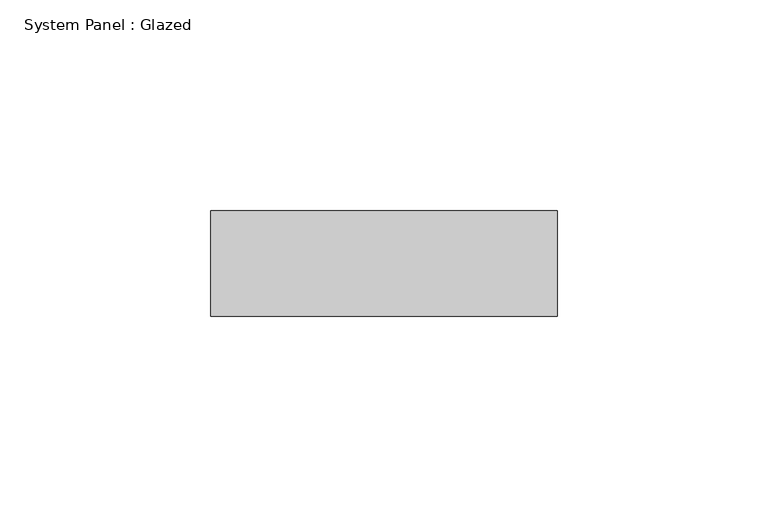
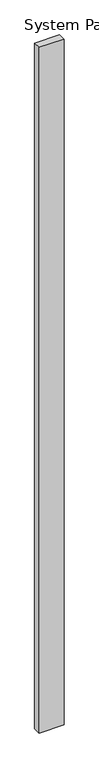
"""IFC4 building model written with IfcOpenShell, lengths in millimetres: plate geometry, System Panel : Glazed."""

from ifc_helpers import new_model, si_unit, origin, origin_with_axes, place, context, project, spatial, polyline, outline, extrude, source, transform, mapped, element, save


def system_panel_glazed_4b83f8e6(model_context):
    return source(origin(), model_context, "Body", "SweptSolid", [
        extrude(outline(polyline([(41.0454544, 24.5), (-41.0454544, 24.5), (-41.0454544, 49.5), (41.0454544, 49.5), (41.0454544, 24.5)])), origin_with_axes(), (0.0, 0.0, 1.0), 2395.0),
    ])


if __name__ == "__main__":
    model = new_model("IFC4")
    model_context = context("Model", 3, world=origin())
    ifc_project = project(units=[si_unit("LENGTHUNIT", "METRE", prefix="MILLI")], contexts=[model_context])
    site = spatial("IfcSite", under=ifc_project)
    building = spatial("IfcBuilding", under=site)
    placement = place(None, origin())
    system_panel_glazed_shape = system_panel_glazed_4b83f8e6(model_context)
    element("IfcPlate", 1, ObjectType="System Panel : Glazed", at=placement, inside=building, context=model_context, shape_type="MappedRepresentation", body=[
        mapped(system_panel_glazed_shape, transform((0.0, 0.0, 0.0), x_axis=(1.0, 0.0, 0.0), y_axis=(0.0, 1.0, 0.0), z_axis=(0.0, 0.0, 1.0))),
    ])
    save(model, "model.ifc")

# Revit data of these elements
# Element 1 (IfcPlate, "System Panel : Glazed")
#   Materials on its faces: "Glass"
# Materials
#   "Glass": class "Glass", colour RGB 218 227 224, transparency 0.85, Description = "Soda Lime Glass", Cost = 0
